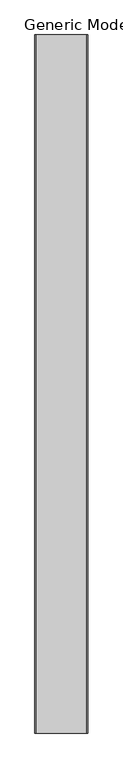
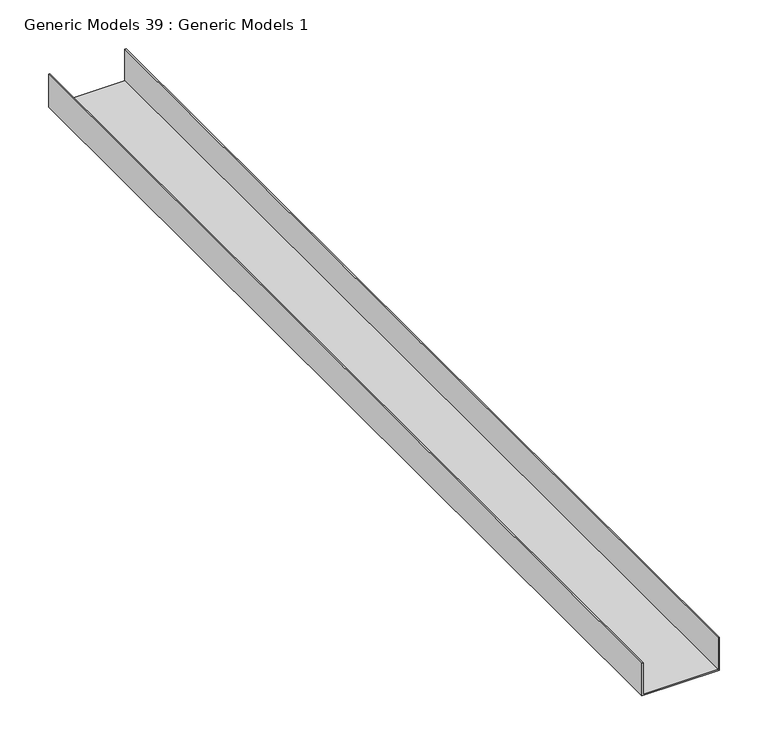
"""IFC4 building model written with IfcOpenShell, lengths in millimetres: proxy geometry, Generic Models 39 : Generic Models 1."""

from ifc_helpers import new_model, si_unit, frame, origin, place, context, project, spatial, polyline, outline, extrude, source, transform, mapped, element, save


def generic_models_39_generic_models_1_ee561edf(model_context):
    return source(origin(), model_context, "Body", "SweptSolid", [
        extrude(outline(polyline([(0.0, 50793.65), (0.0, 50885.725), (41.275, 50885.725), (41.275, 50884.1375), (1.5875, 50884.1375), (1.5875, 50795.2375), (41.275, 50795.2375), (41.275, 50793.65), (0.0, 50793.65)])), frame((0.0, 0.0, 0.0), z_axis=(0.0, 1.0, 0.0), x_axis=(0.0, 0.0, 1.0)), (0.0, 0.0, 1.0), 1219.2),
    ])


if __name__ == "__main__":
    model = new_model("IFC4")
    model_context = context("Model", 3, world=origin())
    ifc_project = project(units=[si_unit("LENGTHUNIT", "METRE", prefix="MILLI")], contexts=[model_context])
    site = spatial("IfcSite", under=ifc_project)
    building = spatial("IfcBuilding", under=site)
    placement = place(None, origin())
    generic_models_39_generic_models_1_shape = generic_models_39_generic_models_1_ee561edf(model_context)
    element("IfcBuildingElementProxy", 1, Name="Generic Models 39 : Generic Models 1", ObjectType="Generic Models 39 : Generic Models 1", at=placement, inside=building, context=model_context, shape_type="MappedRepresentation", body=[
        mapped(generic_models_39_generic_models_1_shape, transform((0.0, 0.0, 0.0), x_axis=(1.0, 0.0, 0.0), y_axis=(0.0, 1.0, 0.0), z_axis=(0.0, 0.0, 1.0))),
    ])
    save(model, "model.ifc")

# Revit data of these elements
# Element 1 (IfcBuildingElementProxy, "Generic Models 39 : Generic Models 1")
#   Materials on its faces: "METAL RUNNER ANCHORED TO STRUCTURE"
# Materials
#   "METAL RUNNER ANCHORED TO STRUCTURE": class "Unassigned", colour RGB 210 209 208, transparency 0, Keynote = "M05121300.02", Cost = 0
